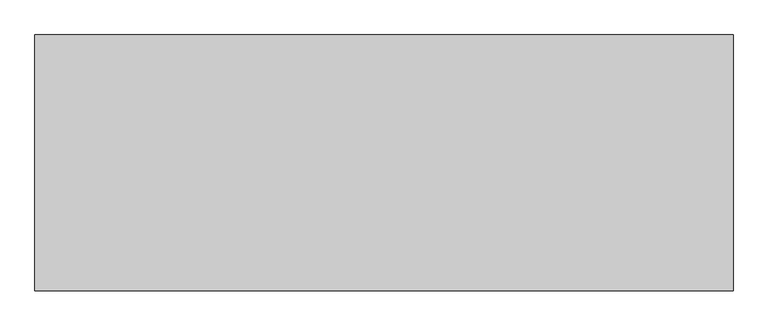
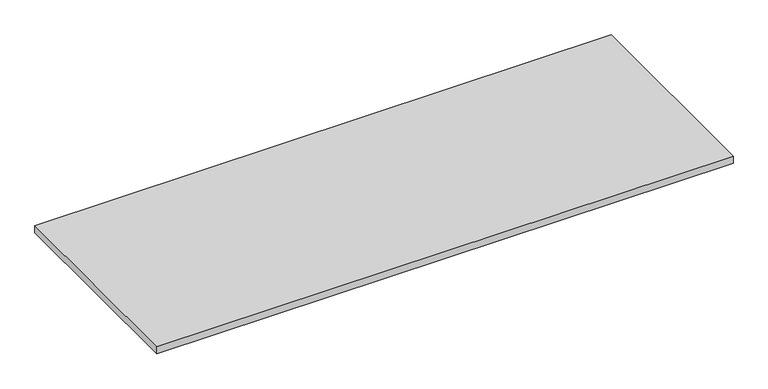
"""IFC4 building model written with IfcOpenShell, lengths in millimetres: proxy geometry, Flooring001 1390 : Flooring001 1390."""

from ifc_helpers import new_model, si_unit, frame, origin, place, context, project, spatial, polyline, outline, extrude, source, transform, mapped, element, save


def generic_models_03f2fe57(model_context):
    return source(origin(), model_context, "Body", "SweptSolid", [
        extrude(outline(polyline([(3694.2883192, 8857.2125834), (3694.2883192, 9590.6375834), (5694.2883192, 9590.6375834), (5694.2883192, 8857.2125834), (3694.2883192, 8857.2125834)])), frame((0.0, 0.0, 36556.696), z_axis=(0.0, 0.0, 1.0), x_axis=(1.0, 0.0, 0.0)), (0.0, 0.0, 1.0), 25.4),
    ])


if __name__ == "__main__":
    model = new_model("IFC4")
    model_context = context("Model", 3, world=origin())
    ifc_project = project(units=[si_unit("LENGTHUNIT", "METRE", prefix="MILLI")], contexts=[model_context])
    site = spatial("IfcSite", under=ifc_project)
    building = spatial("IfcBuilding", under=site)
    placement = place(None, origin())
    generic_models_shape = generic_models_03f2fe57(model_context)
    element("IfcBuildingElementProxy", 1, Name="Flooring001 1390 : Flooring001 1390", ObjectType="Flooring001 1390 : Flooring001 1390", at=placement, inside=building, context=model_context, shape_type="MappedRepresentation", body=[
        mapped(generic_models_shape, transform((0.0, 0.0, 0.0), x_axis=(1.0, 0.0, 0.0), y_axis=(0.0, 1.0, 0.0), z_axis=(0.0, 0.0, 1.0))),
    ])
    save(model, "model.ifc")

# Revit data of these elements
# Type "Flooring001 1390 : Flooring001 1390"
#   NameOverride = "Flooring001"
# Element 1 (IfcBuildingElementProxy, "Flooring001 1390 : Flooring001 1390")
#   Materials on its faces: "WOOD FLOORING (SPEC TBD)"
# Materials
#   "WOOD FLOORING (SPEC TBD)": class "Unassigned", colour RGB 201 162 125, transparency 0
